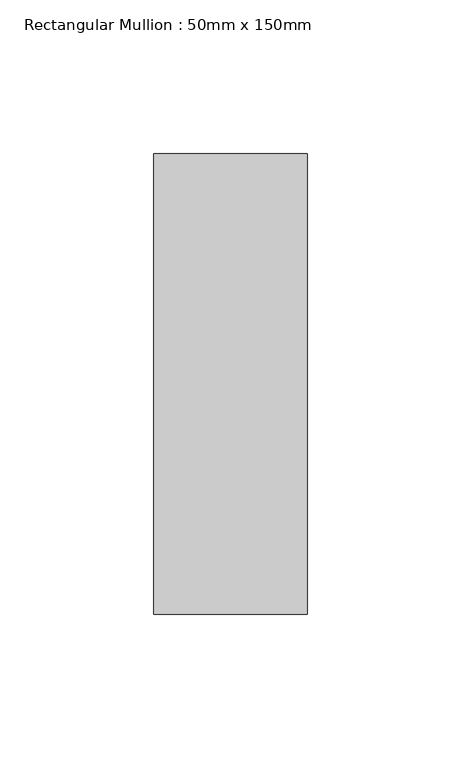
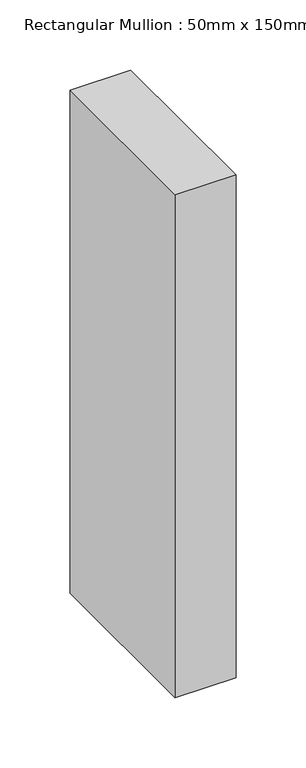
"""IFC4 building model written with IfcOpenShell, lengths in millimetres: member geometry, Rectangular Mullion : 50mm x 150mm."""

from ifc_helpers import new_model, si_unit, frame, origin, place, context, project, spatial, polyline, outline, extrude, source, transform, mapped, element, save


def rectangular_mullion_50mm_x_150mm_f27418de(model_context):
    return source(origin(), model_context, "Body", "SweptSolid", [
        extrude(outline(polyline([(0.0, 75.0), (0.0, -75.0), (-50.0, -75.0), (-50.0, 75.0), (0.0, 75.0)])), frame((0.0, 0.0, -437.8787879), z_axis=(0.0, 0.0, 1.0), x_axis=(1.0, 0.0, 0.0)), (0.0, 0.0, 1.0), 437.8787879),
    ])


if __name__ == "__main__":
    model = new_model("IFC4")
    model_context = context("Model", 3, world=origin())
    ifc_project = project(units=[si_unit("LENGTHUNIT", "METRE", prefix="MILLI")], contexts=[model_context])
    site = spatial("IfcSite", under=ifc_project)
    building = spatial("IfcBuilding", under=site)
    placement = place(None, origin())
    rectangular_mullion_50mm_x_150mm_shape = rectangular_mullion_50mm_x_150mm_f27418de(model_context)
    element("IfcMember", 1, ObjectType="Rectangular Mullion : 50mm x 150mm", at=placement, inside=building, context=model_context, shape_type="MappedRepresentation", body=[
        mapped(rectangular_mullion_50mm_x_150mm_shape, transform((0.0, 0.0, 0.0), x_axis=(1.0, 0.0, 0.0), y_axis=(0.0, 1.0, 0.0), z_axis=(0.0, 0.0, 1.0))),
    ])
    save(model, "model.ifc")

# Revit data of these elements
# Type "Rectangular Mullion : 50mm x 150mm"
#   built-in parameter 1007304 = 0.492126 (stored number, unit not read)
#   built-in parameter 1007301 = 0.082021 (stored number, unit not read)
#   built-in parameter 1007300 = 0.082021 (stored number, unit not read)
# Element 1 (IfcMember, "Rectangular Mullion : 50mm x 150mm")
#   Materials on its faces: "Aluminum"
# Materials
#   "Aluminum": class "Metal", colour RGB 244 244 244, transparency 0, Description = "Aluminum 6061", Cost = 0
